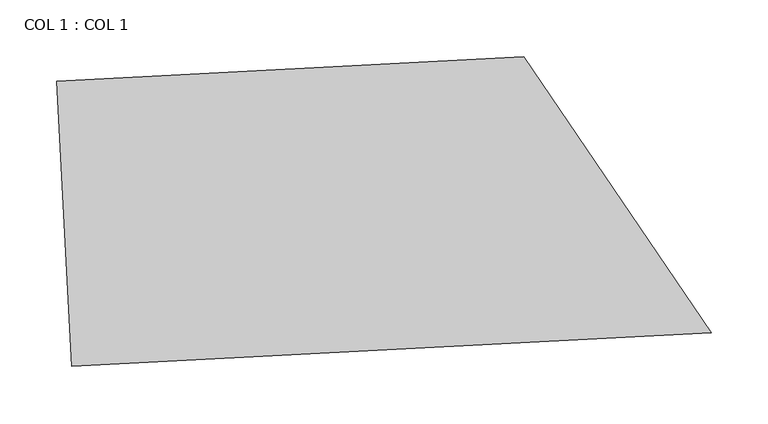
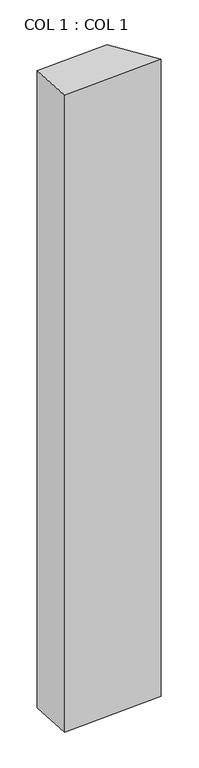
"""IFC4 building model written with IfcOpenShell, lengths in millimetres: column geometry, COL 1 : COL 1."""

import ifcopenshell
import ifcopenshell.guid

model = None  # the IFC model being written
_history = None  # IfcOwnerHistory: only IFC2X3 demands one
_inside = {}  # id of a spatial element -> (the spatial element, [elements in it])
_under = {}  # id of a project, library or spatial element -> (it, [spatial elements below it])
_declared = {}  # id of a project -> (the project, [libraries it declares])
_typed = {}  # id of a type object -> (the type object, [elements of that type])
_made_of = {}  # id of a material, layer set ... -> (it, [elements and type objects made of it])


def new_model(schema):
    """Start an empty IFC model of exactly this schema.

    Asked for "IFC4X3", IfcOpenShell would pick the latest addendum, in which some entities
    have other attributes; the version numbers below select the first issue.
    IFC2X3 requires an IfcOwnerHistory on every rooted entity: one is made here for all.
    """
    global model, _history
    if schema == "IFC4X3":
        model = ifcopenshell.file(schema_version=(4, 3, 0, 0))
    else:
        model = ifcopenshell.file(schema=schema)
    _inside.clear()
    _under.clear()
    _declared.clear()
    _typed.clear()
    _made_of.clear()
    _history = None
    if model.schema == "IFC2X3":
        org = make("IfcOrganization", Name="unknown")
        user = make(
            "IfcPersonAndOrganization",
            ThePerson=make("IfcPerson", FamilyName="unknown"),
            TheOrganization=org,
        )
        app = make(
            "IfcApplication",
            ApplicationDeveloper=org,
            Version="unknown",
            ApplicationFullName="unknown",
            ApplicationIdentifier="unknown",
        )
        _history = make(
            "IfcOwnerHistory",
            OwningUser=user,
            OwningApplication=app,
            ChangeAction="ADDED",
            CreationDate=0,
        )
    return model


def make(cls, **values):
    """One entity of the class cls with the attributes given. An attribute that is None is left unset."""
    return model.create_entity(
        cls, **{name: value for name, value in values.items() if value is not None}
    )


def rooted(cls, **values):
    """An entity with a GlobalId (a new one), such as an element, a storey or a relation."""
    return make(cls, GlobalId=ifcopenshell.guid.new(), OwnerHistory=_history, **values)


def si_unit(unit_type, name, prefix=None):
    """IfcSIUnit, for example si_unit("LENGTHUNIT", "METRE", prefix="MILLI")."""
    return make("IfcSIUnit", UnitType=unit_type, Prefix=prefix, Name=name)


def assignment(units):
    """IfcUnitAssignment: the units of a project."""
    return None if units is None else make("IfcUnitAssignment", Units=units)


def point(xyz):
    """IfcCartesianPoint."""
    return None if xyz is None else make("IfcCartesianPoint", Coordinates=xyz)


def direction(xyz):
    """IfcDirection."""
    return None if xyz is None else make("IfcDirection", DirectionRatios=xyz)


def frame(location, z_axis=None, x_axis=None):
    """IfcAxis2Placement3D, a coordinate frame: its origin and axes. An axis left out is left unset."""
    return make(
        "IfcAxis2Placement3D",
        Location=point(location),
        Axis=direction(z_axis),
        RefDirection=direction(x_axis),
    )


def frame_2d(location, x_axis=None):
    """IfcAxis2Placement2D, a coordinate frame in the plane: its origin and x axis."""
    return make(
        "IfcAxis2Placement2D", Location=point(location), RefDirection=direction(x_axis)
    )


def origin():
    """The frame at (0, 0, 0) with its axes left unset."""
    return frame((0.0, 0.0, 0.0))


def origin_with_axes():
    """The frame at (0, 0, 0) with the z axis (0, 0, 1) and the x axis (1, 0, 0) written out."""
    return frame((0.0, 0.0, 0.0), z_axis=(0.0, 0.0, 1.0), x_axis=(1.0, 0.0, 0.0))


def place(relative_to, where):
    """IfcLocalPlacement: puts the frame where relative to a parent placement (None: the world)."""
    return make(
        "IfcLocalPlacement", PlacementRelTo=relative_to, RelativePlacement=where
    )


def context(
    kind, dimensions, precision=None, world=None, true_north=None, identifier=None
):
    """IfcGeometricRepresentationContext, for example the 3D "Model" context."""
    return make(
        "IfcGeometricRepresentationContext",
        ContextIdentifier=identifier,
        ContextType=kind,
        CoordinateSpaceDimension=dimensions,
        Precision=precision,
        WorldCoordinateSystem=world,
        TrueNorth=true_north,
    )


def project(units=None, contexts=None):
    """IfcProject with its units and contexts."""
    return rooted(
        "IfcProject",
        Name="project",
        RepresentationContexts=contexts,
        UnitsInContext=assignment(units),
    )


def spatial(cls, under=None, at=None, **own):
    """A site, building, storey or space (cls), placed at a placement, below another one or the project."""
    s = rooted(cls, ObjectPlacement=at, **own)
    if under is not None:
        _under.setdefault(under.id(), (under, []))[1].append(s)
    return s


def polyline(points):
    """IfcPolyline through the points."""
    return make("IfcPolyline", Points=[point(p) for p in points])


def circle_curve(where, radius):
    """IfcCircle in the frame where."""
    return make("IfcCircle", Position=where, Radius=radius)


def trimmed(basis, trim1, trim2, sense, master):
    """IfcTrimmedCurve: the piece of a basis curve between two trims."""
    return make(
        "IfcTrimmedCurve",
        BasisCurve=basis,
        Trim1=trim1,
        Trim2=trim2,
        SenseAgreement=sense,
        MasterRepresentation=master,
    )


def segment(curve, same_sense, transition):
    """IfcCompositeCurveSegment."""
    return make(
        "IfcCompositeCurveSegment",
        Transition=transition,
        SameSense=same_sense,
        ParentCurve=curve,
    )


def composite_curve(segments, self_intersect=None):
    """IfcCompositeCurve: segments joined end to end."""
    return make("IfcCompositeCurve", Segments=segments, SelfIntersect=self_intersect)


def outline(outer, holes=None, kind="AREA"):
    """IfcArbitraryClosedProfileDef: a profile drawn as a closed curve; with holes, ...WithVoids."""
    if holes is None:
        return make("IfcArbitraryClosedProfileDef", ProfileType=kind, OuterCurve=outer)
    return make(
        "IfcArbitraryProfileDefWithVoids",
        ProfileType=kind,
        OuterCurve=outer,
        InnerCurves=holes,
    )


def extrude(swept, where, along, depth):
    """IfcExtrudedAreaSolid: the profile swept, set in the frame where, extruded along a direction by depth."""
    return make(
        "IfcExtrudedAreaSolid",
        SweptArea=swept,
        Position=where,
        ExtrudedDirection=direction(along),
        Depth=depth,
    )


def shape(context_of_items, identifier, shape_type, items):
    """IfcShapeRepresentation: the items that make up one representation, for example the "Body"."""
    return make(
        "IfcShapeRepresentation",
        ContextOfItems=context_of_items,
        RepresentationIdentifier=identifier,
        RepresentationType=shape_type,
        Items=items,
    )


def source(mapping_origin, context_of_items, identifier, shape_type, items):
    """IfcRepresentationMap: a shape defined once, which mapped items show again and again."""
    return make(
        "IfcRepresentationMap",
        MappingOrigin=mapping_origin,
        MappedRepresentation=shape(context_of_items, identifier, shape_type, items),
    )


def transform(
    local_origin,
    x_axis=None,
    y_axis=None,
    z_axis=None,
    scale=None,
    scale2=None,
    scale3=None,
    uniform=True,
):
    """IfcCartesianTransformationOperator3D, or its non-uniform kind. x_axis, y_axis, z_axis: its Axis1, 2, 3."""
    if uniform:
        return make(
            "IfcCartesianTransformationOperator3D",
            Axis1=direction(x_axis),
            Axis2=direction(y_axis),
            LocalOrigin=point(local_origin),
            Scale=scale,
            Axis3=direction(z_axis),
        )
    return make(
        "IfcCartesianTransformationOperator3DnonUniform",
        Axis1=direction(x_axis),
        Axis2=direction(y_axis),
        LocalOrigin=point(local_origin),
        Scale=scale,
        Axis3=direction(z_axis),
        Scale2=scale2,
        Scale3=scale3,
    )


def mapped(mapping_source, mapping_target):
    """IfcMappedItem: shows the shape of a source again, moved by a transform."""
    return make(
        "IfcMappedItem", MappingSource=mapping_source, MappingTarget=mapping_target
    )


def made_of(thing, what):
    """Note that an element or type object is made of a material, layer set ...; save() writes the relation."""
    if what is not None:
        _made_of.setdefault(what.id(), (what, []))[1].append(thing)
    return thing


def element(
    cls,
    number,
    at=None,
    inside=None,
    cuts=None,
    type_object=None,
    material=None,
    context=None,
    identifier="Body",
    shape_type=None,
    held_by="IfcProductDefinitionShape",
    body=None,
    shapes=None,
    **own,
):
    """One element of the class cls, such as IfcWall. Its Tag is "e" and its number.

    at: its placement. inside: the storey or other place that contains it. cuts: it is an
    opening in that element (IfcRelVoidsElement). A single representation is given by context,
    identifier, shape_type and body (its items); several are given by shapes. held_by: the class
    of the entity that holds the representations. save() writes the other relations.
    """
    e = rooted(cls, Tag="e%d" % number, ObjectPlacement=at, **own)
    if body is not None:
        shapes = [shape(context, identifier, shape_type, body)]
    if shapes is not None:
        e.Representation = make(held_by, Representations=shapes)
    if inside is not None:
        _inside.setdefault(inside.id(), (inside, []))[1].append(e)
    if cuts is not None:
        rooted(
            "IfcRelVoidsElement", RelatingBuildingElement=cuts, RelatedOpeningElement=e
        )
    if type_object is not None:
        _typed.setdefault(type_object.id(), (type_object, []))[1].append(e)
    return made_of(e, material)


def aggregate(whole, parts):
    """IfcRelAggregates: a whole, such as a stair, and the parts it consists of."""
    return rooted("IfcRelAggregates", RelatingObject=whole, RelatedObjects=parts)


def save(model, path):
    """Write the relations noted so far, then the file.

    IfcRelAggregates (storeys below a building ...), IfcRelContainedInSpatialStructure (elements
    in a storey), IfcRelDefinesByType, IfcRelAssociatesMaterial and IfcRelDeclares: one each for
    every whole, place, type object, material and project.
    """
    for whole, parts in _under.values():
        aggregate(whole, parts)
    for where, things in _inside.values():
        rooted(
            "IfcRelContainedInSpatialStructure",
            RelatedElements=things,
            RelatingStructure=where,
        )
    for kind, things in _typed.values():
        rooted("IfcRelDefinesByType", RelatedObjects=things, RelatingType=kind)
    for what, things in _made_of.values():
        rooted("IfcRelAssociatesMaterial", RelatedObjects=things, RelatingMaterial=what)
    for by, libraries in _declared.values():
        rooted("IfcRelDeclares", RelatingContext=by, RelatedDefinitions=libraries)
    model.write(path)


def col_1_col_1_626721b3(model_context):
    return source(origin(), model_context, "Body", "SweptSolid", [
        extrude(outline(composite_curve([segment(polyline([(6345.0539916, -30821.1600547), (6755.6659066, -30799.6407961)]), True, "CONTINUOUS"), segment(trimmed(circle_curve(frame_2d((3840.295048, -32955.4239436)), 3625.85), [point((6755.6659066, -30799.6407961))], [point((6920.2784026, -31042.1830394))], False, "CARTESIAN"), True, "CONTINUOUS"), segment(polyline([(6920.2784026, -31042.1830394), (6358.1811578, -31071.6413077), (6345.0539916, -30821.1600547)]), True, "CONTINUOUS")], self_intersect=False)), origin_with_axes(), (0.0, 0.0, 1.0), 3810.0),
    ])


if __name__ == "__main__":
    model = new_model("IFC4")
    model_context = context("Model", 3, world=origin())
    ifc_project = project(units=[si_unit("LENGTHUNIT", "METRE", prefix="MILLI")], contexts=[model_context])
    site = spatial("IfcSite", under=ifc_project)
    building = spatial("IfcBuilding", under=site)
    placement = place(None, origin())
    col_1_col_1_shape = col_1_col_1_626721b3(model_context)
    element("IfcColumn", 1, ObjectType="COL 1 : COL 1", at=placement, inside=building, context=model_context, shape_type="MappedRepresentation", body=[
        mapped(col_1_col_1_shape, transform((0.0, 0.0, 0.0), x_axis=(1.0, 0.0, 0.0), y_axis=(0.0, 1.0, 0.0), z_axis=(0.0, 0.0, 1.0))),
    ])
    save(model, "model.ifc")

# Revit data of these elements
# Element 1 (IfcColumn, "COL 1 : COL 1")
#   Materials on its faces: "Default Wall"
# Materials
#   "Default Wall": class "Miscellaneous", colour RGB 128 128 128, transparency 0
